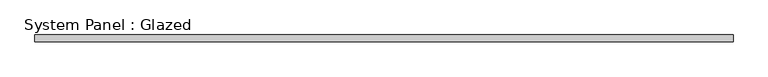
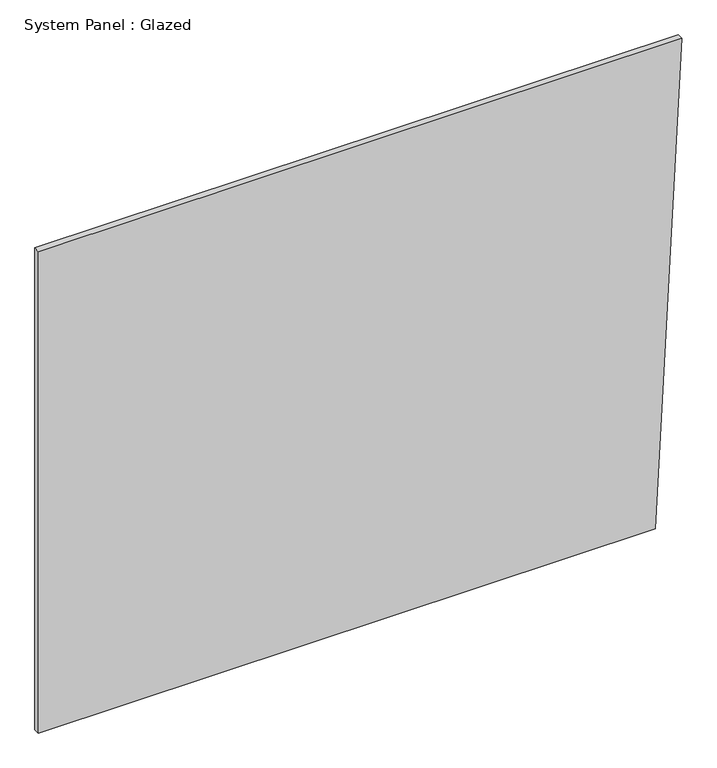
"""IFC4 building model written with IfcOpenShell, lengths in millimetres: plate geometry, System Panel : Glazed."""

from ifc_helpers import new_model, si_unit, frame, origin, place, context, project, spatial, polyline, outline, extrude, source, transform, mapped, element, save


def system_panel_glazed_f6a0a944(model_context):
    return source(origin(), model_context, "Body", "SweptSolid", [
        extrude(outline(polyline([(0.0, -1317.8741594), (0.0, 1208.7338763), (2085.3785982, 1317.8741594), (2085.3785982, -1317.8741594), (0.0, -1317.8741594)])), frame((0.0, -44.45, 0.0), z_axis=(0.0, 1.0, 0.0), x_axis=(0.0, 0.0, 1.0)), (0.0, 0.0, 1.0), 25.4),
    ])


if __name__ == "__main__":
    model = new_model("IFC4")
    model_context = context("Model", 3, world=origin())
    ifc_project = project(units=[si_unit("LENGTHUNIT", "METRE", prefix="MILLI")], contexts=[model_context])
    site = spatial("IfcSite", under=ifc_project)
    building = spatial("IfcBuilding", under=site)
    placement = place(None, origin())
    system_panel_glazed_shape = system_panel_glazed_f6a0a944(model_context)
    element("IfcPlate", 1, ObjectType="System Panel : Glazed", at=placement, inside=building, context=model_context, shape_type="MappedRepresentation", body=[
        mapped(system_panel_glazed_shape, transform((0.0, 0.0, 0.0), x_axis=(1.0, 0.0, 0.0), y_axis=(0.0, 1.0, 0.0), z_axis=(0.0, 0.0, 1.0))),
    ])
    save(model, "model.ifc")

# Revit data of these elements
# Type "System Panel : Glazed"
#   Construction Type Id = "GSP4R"
#   Analytic Construction = "1/8 in Pilkington single glazing"
#   Visual Light Transmittance = 0.9
#   Solar Heat Gain Coefficient = 0.86
#   Heat Transfer Coefficient (U) = 1.18115 BTU/(h·ft²·°F)
#   Define Thermal Properties by = 1
# Element 1 (IfcPlate, "System Panel : Glazed")
#   Materials on its faces: "Glass"
# Materials
#   "Glass": class "Glass", colour RGB 0 128 192, transparency 0.75, Description = "Soda Lime Glass", Cost = 0
